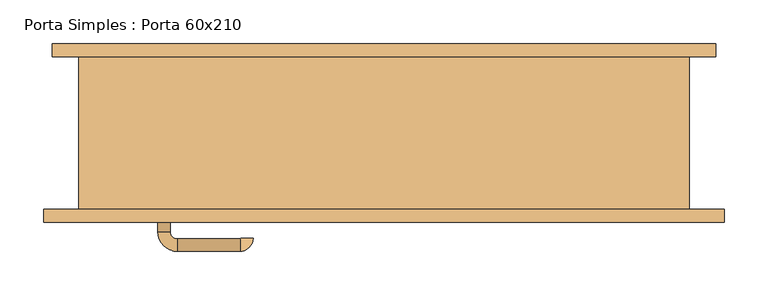
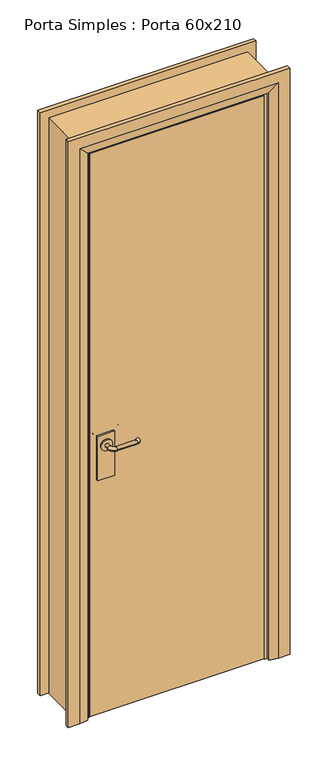
"""IFC4 building model written with IfcOpenShell, lengths in millimetres: door geometry, Porta Simples : Porta 60x210."""

from ifc_helpers import new_model, si_unit, point, frame, frame_2d, origin, place, context, project, spatial, polyline, circle_curve, ellipse_curve, trimmed, segment, composite_curve, outline, extrude, faceted_brep, source, transform, mapped, element, save
from ifc_brep_helpers import plane_surface, cylinder_surface, revolved_surface, advanced_brep


def porta_simples_porta_60x210_4542fb52(model_context):
    return source(origin(), model_context, "Body", "SolidModel", [
        extrude(outline(composite_curve([segment(trimmed(circle_curve(frame_2d((1050.0, -252.0)), 20.0), [point((1050.0, -272.0))], [point((1050.0, -232.0))], False, "CARTESIAN"), True, "CONTINUOUS"), segment(trimmed(circle_curve(frame_2d((1050.0, -252.0)), 20.0), [point((1050.0, -232.0))], [point((1050.0, -272.0))], False, "CARTESIAN"), True, "CONTINUOUS")], self_intersect=False)), frame((0.0, -46.3, 0.0), z_axis=(0.0, 1.0, 0.0), x_axis=(0.0, 0.0, 1.0)), (0.0, 0.0, 1.0), 4.5929895),
        advanced_brep(
        [(-245.0, -41.7070105, 1050.0), (-259.0, -41.7070105, 1050.0), (-245.0, -26.3, 1050.0), (-259.0, -26.3, 1050.0), (-237.0, -4.3, 1050.0), (-237.0, -18.3, 1050.0), (-165.0, -18.3, 1050.0), (-165.0, -4.3, 1050.0), (-164.0, -19.3, 1050.0), (-150.0, -19.3, 1050.0)],
        [
            (0, 1, circle_curve(frame((-252.0, -41.7070105, 1050.0), z_axis=(0.0, -1.0, 0.0), x_axis=(-1.0, 0.0, 0.0)), 7.0)),
            (1, 0, circle_curve(frame((-252.0, -41.7070105, 1050.0), z_axis=(0.0, -1.0, 0.0), x_axis=(-1.0, 0.0, 0.0)), 7.0)),
            (0, 2),
            (2, 3, circle_curve(frame((-252.0, -26.3, 1050.0), z_axis=(0.0, -1.0, 0.0), x_axis=(-1.0, 0.0, 0.0)), 7.0)),
            (3, 1),
            (3, 2, circle_curve(frame((-252.0, -26.3, 1050.0), z_axis=(0.0, -1.0, 0.0), x_axis=(-1.0, 0.0, 0.0)), 7.0)),
            (4, 3, circle_curve(frame((-237.0, -26.3, 1050.0), z_axis=(0.0, 0.0, 1.0), x_axis=(-1.0, 0.0, 0.0)), 22.0)),
            (2, 5, circle_curve(frame((-237.0, -26.3, 1050.0), z_axis=(0.0, 0.0, -1.0), x_axis=(-1.0, 0.0, 0.0)), 8.0)),
            (5, 4, circle_curve(frame((-237.0, -11.3, 1050.0), z_axis=(-1.0, 0.0, 0.0), x_axis=(0.0, 1.0, 0.0)), 7.0)),
            (4, 5, circle_curve(frame((-237.0, -11.3, 1050.0), z_axis=(-1.0, 0.0, 0.0), x_axis=(0.0, 1.0, 0.0)), 7.0)),
            (5, 6),
            (6, 7, circle_curve(frame((-165.0, -11.3, 1050.0), z_axis=(-1.0, 0.0, 0.0), x_axis=(0.0, 1.0, 0.0)), 7.0)),
            (7, 4),
            (7, 6, circle_curve(frame((-165.0, -11.3, 1050.0), z_axis=(-1.0, 0.0, 0.0), x_axis=(0.0, 1.0, 0.0)), 7.0)),
            (8, 9, circle_curve(frame((-157.0, -19.3, 1050.0), z_axis=(0.0, -1.0, 0.0), x_axis=(1.0, 0.0, 0.0)), 7.0)),
            (9, 8, circle_curve(frame((-157.0, -19.3, 1050.0), z_axis=(0.0, -1.0, 0.0), x_axis=(1.0, 0.0, 0.0)), 7.0)),
            (9, 7, circle_curve(frame((-165.0, -19.3, 1050.0), z_axis=(0.0, 0.0, 1.0), x_axis=(0.0, 1.0, 0.0)), 15.0)),
            (6, 8, circle_curve(frame((-165.0, -19.3, 1050.0), z_axis=(0.0, 0.0, -1.0), x_axis=(0.0, 1.0, 0.0)), 1.0)),
        ],
        [
            plane_surface(frame((-252.0, -41.7070105, 1050.0), z_axis=(0.0, -1.0, 0.0), x_axis=(0.0, 0.0, 1.0))),
            cylinder_surface(frame((-252.0, -41.7070105, 1050.0), z_axis=(0.0, -1.0, 0.0), x_axis=(-1.0, 0.0, 0.0)), 7.0),
            revolved_surface(trimmed(ellipse_curve(frame((-252.0, -26.3, 1050.0), z_axis=(0.0, -1.0, 0.0), x_axis=(-1.0, 0.0, 0.0)), 7.0, 7.0), [point((-245.0, -26.3, 1050.0))], [point((-259.0, -26.3, 1050.0))], True, "CARTESIAN"), (-237.0, -26.3, 1050.0), (0.0, 0.0, -1.0)),
            revolved_surface(trimmed(ellipse_curve(frame((-252.0, -26.3, 1050.0), z_axis=(0.0, -1.0, 0.0), x_axis=(-1.0, 0.0, 0.0)), 7.0, 7.0), [point((-259.0, -26.3, 1050.0))], [point((-245.0, -26.3, 1050.0))], True, "CARTESIAN"), (-237.0, -26.3, 1050.0), (0.0, 0.0, -1.0)),
            cylinder_surface(frame((-237.0, -11.3, 1050.0), z_axis=(-1.0, 0.0, 0.0), x_axis=(0.0, 1.0, 0.0)), 7.0),
            plane_surface(frame((-157.0, -19.3, 1050.0), z_axis=(0.0, -1.0, 0.0), x_axis=(0.0, 0.0, 1.0))),
            revolved_surface(trimmed(ellipse_curve(frame((-165.0, -11.3, 1050.0), z_axis=(-1.0, 0.0, 0.0), x_axis=(0.0, 1.0, 0.0)), 7.0, 7.0), [point((-165.0, -18.3, 1050.0))], [point((-165.0, -4.3, 1050.0))], True, "CARTESIAN"), (-165.0, -19.3, 1050.0), (0.0, 0.0, -1.0)),
            revolved_surface(trimmed(ellipse_curve(frame((-165.0, -11.3, 1050.0), z_axis=(-1.0, 0.0, 0.0), x_axis=(0.0, 1.0, 0.0)), 7.0, 7.0), [point((-165.0, -4.3, 1050.0))], [point((-165.0, -18.3, 1050.0))], True, "CARTESIAN"), (-165.0, -19.3, 1050.0), (0.0, 0.0, -1.0)),
        ],
        [
            (0, [[1, 2]]),
            (1, [[-1, 3, 4, 5]]),
            (1, [[-2, -5, 6, -3]]),
            (2, [[7, -4, 8, 9]]),
            (3, [[-8, -6, -7, 10]]),
            (4, [[-9, 11, 12, 13]]),
            (4, [[-10, -13, 14, -11]]),
            (5, [[15, 16]]),
            (6, [[17, -12, 18, -16]]),
            (7, [[-18, -14, -17, -15]]),
        ],
    ),
        extrude(outline(polyline([(-222.0, -52.3), (-282.0, -52.3), (-282.0, -46.3), (-222.0, -46.3), (-222.0, -52.3)])), frame((0.0, 0.0, 925.0), z_axis=(0.0, 0.0, 1.0), x_axis=(1.0, 0.0, 0.0)), (0.0, 0.0, 1.0), 165.0),
        extrude(outline(composite_curve([segment(trimmed(circle_curve(frame_2d((1050.0, -252.0)), 20.0), [point((1050.0, -272.0))], [point((1050.0, -232.0))], False, "CARTESIAN"), True, "CONTINUOUS"), segment(trimmed(circle_curve(frame_2d((1050.0, -252.0)), 20.0), [point((1050.0, -232.0))], [point((1050.0, -272.0))], False, "CARTESIAN"), True, "CONTINUOUS")], self_intersect=False)), frame((0.0, -97.8929895, 0.0), z_axis=(0.0, 1.0, 0.0), x_axis=(0.0, 0.0, 1.0)), (0.0, 0.0, 1.0), 4.5929895),
        advanced_brep(
        [(-245.0, -97.8929895, 1050.0), (-259.0, -97.8929895, 1050.0), (-259.0, -113.3, 1050.0), (-245.0, -113.3, 1050.0), (-237.0, -135.3, 1050.0), (-237.0, -121.3, 1050.0), (-165.0, -135.3, 1050.0), (-165.0, -121.3, 1050.0), (-164.0, -120.3, 1050.0), (-150.0, -120.3, 1050.0)],
        [
            (0, 1, circle_curve(frame((-252.0, -97.8929895, 1050.0), z_axis=(0.0, 1.0, 0.0), x_axis=(-1.0, 0.0, 0.0)), 7.0)),
            (1, 0, circle_curve(frame((-252.0, -97.8929895, 1050.0), z_axis=(0.0, 1.0, 0.0), x_axis=(-1.0, 0.0, 0.0)), 7.0)),
            (1, 2),
            (2, 3, circle_curve(frame((-252.0, -113.3, 1050.0), z_axis=(0.0, 1.0, 0.0), x_axis=(-1.0, 0.0, 0.0)), 7.0)),
            (3, 0),
            (3, 2, circle_curve(frame((-252.0, -113.3, 1050.0), z_axis=(0.0, 1.0, 0.0), x_axis=(-1.0, 0.0, 0.0)), 7.0)),
            (4, 5, circle_curve(frame((-237.0, -128.3, 1050.0), z_axis=(-1.0, 0.0, 0.0), x_axis=(0.0, -1.0, 0.0)), 7.0)),
            (5, 3, circle_curve(frame((-237.0, -113.3, 1050.0), z_axis=(0.0, 0.0, -1.0), x_axis=(-1.0, 0.0, 0.0)), 8.0)),
            (2, 4, circle_curve(frame((-237.0, -113.3, 1050.0), z_axis=(0.0, 0.0, 1.0), x_axis=(-1.0, 0.0, 0.0)), 22.0)),
            (5, 4, circle_curve(frame((-237.0, -128.3, 1050.0), z_axis=(-1.0, 0.0, 0.0), x_axis=(0.0, -1.0, 0.0)), 7.0)),
            (4, 6),
            (6, 7, circle_curve(frame((-165.0, -128.3, 1050.0), z_axis=(-1.0, 0.0, 0.0), x_axis=(0.0, -1.0, 0.0)), 7.0)),
            (7, 5),
            (7, 6, circle_curve(frame((-165.0, -128.3, 1050.0), z_axis=(-1.0, 0.0, 0.0), x_axis=(0.0, -1.0, 0.0)), 7.0)),
            (8, 9, circle_curve(frame((-157.0, -120.3, 1050.0), z_axis=(0.0, 1.0, 0.0), x_axis=(1.0, 0.0, 0.0)), 7.0)),
            (9, 8, circle_curve(frame((-157.0, -120.3, 1050.0), z_axis=(0.0, 1.0, 0.0), x_axis=(1.0, 0.0, 0.0)), 7.0)),
            (8, 7, circle_curve(frame((-165.0, -120.3, 1050.0), z_axis=(0.0, 0.0, -1.0), x_axis=(0.0, -1.0, 0.0)), 1.0)),
            (6, 9, circle_curve(frame((-165.0, -120.3, 1050.0), z_axis=(0.0, 0.0, 1.0), x_axis=(0.0, -1.0, 0.0)), 15.0)),
        ],
        [
            plane_surface(frame((-252.0, -97.8929895, 1050.0), z_axis=(0.0, 1.0, 0.0), x_axis=(0.0, 0.0, 1.0))),
            cylinder_surface(frame((-252.0, -97.8929895, 1050.0), z_axis=(0.0, 1.0, 0.0), x_axis=(-1.0, 0.0, 0.0)), 7.0),
            revolved_surface(trimmed(ellipse_curve(frame((-252.0, -113.3, 1050.0), z_axis=(0.0, -1.0, 0.0), x_axis=(-1.0, 0.0, 0.0)), 7.0, 7.0), [point((-245.0, -113.3, 1050.0))], [point((-259.0, -113.3, 1050.0))], True, "CARTESIAN"), (-237.0, -113.3, 1050.0), (0.0, 0.0, -1.0)),
            revolved_surface(trimmed(ellipse_curve(frame((-252.0, -113.3, 1050.0), z_axis=(0.0, -1.0, 0.0), x_axis=(-1.0, 0.0, 0.0)), 7.0, 7.0), [point((-259.0, -113.3, 1050.0))], [point((-245.0, -113.3, 1050.0))], True, "CARTESIAN"), (-237.0, -113.3, 1050.0), (0.0, 0.0, -1.0)),
            cylinder_surface(frame((-237.0, -128.3, 1050.0), z_axis=(-1.0, 0.0, 0.0), x_axis=(0.0, -1.0, 0.0)), 7.0),
            plane_surface(frame((-157.0, -120.3, 1050.0), z_axis=(0.0, 1.0, 0.0), x_axis=(0.0, 0.0, 1.0))),
            revolved_surface(trimmed(ellipse_curve(frame((-165.0, -128.3, 1050.0), z_axis=(1.0, 0.0, 0.0), x_axis=(0.0, -1.0, 0.0)), 7.0, 7.0), [point((-165.0, -121.3, 1050.0))], [point((-165.0, -135.3, 1050.0))], True, "CARTESIAN"), (-165.0, -120.3, 1050.0), (0.0, 0.0, -1.0)),
            revolved_surface(trimmed(ellipse_curve(frame((-165.0, -128.3, 1050.0), z_axis=(1.0, 0.0, 0.0), x_axis=(0.0, -1.0, 0.0)), 7.0, 7.0), [point((-165.0, -135.3, 1050.0))], [point((-165.0, -121.3, 1050.0))], True, "CARTESIAN"), (-165.0, -120.3, 1050.0), (0.0, 0.0, -1.0)),
        ],
        [
            (0, [[1, 2]]),
            (1, [[3, 4, 5, -2]]),
            (1, [[-5, 6, -3, -1]]),
            (2, [[7, 8, -4, 9]]),
            (3, [[10, -9, -6, -8]]),
            (4, [[11, 12, 13, -7]]),
            (4, [[-13, 14, -11, -10]]),
            (5, [[15, 16]]),
            (6, [[-15, 17, -12, 18]]),
            (7, [[-16, -18, -14, -17]]),
        ],
    ),
        extrude(outline(polyline([(-222.0, -87.3), (-222.0, -93.3), (-282.0, -93.3), (-282.0, -87.3), (-222.0, -87.3)])), frame((0.0, 0.0, 925.0), z_axis=(0.0, 0.0, 1.0), x_axis=(1.0, 0.0, 0.0)), (0.0, 0.0, 1.0), 165.0),
        extrude(outline(polyline([(307.0, -52.3), (307.0, -87.3), (-307.0, -87.3), (-307.0, -52.3), (307.0, -52.3)])), frame((0.0, 0.0, 53.0), z_axis=(0.0, 0.0, 1.0), x_axis=(1.0, 0.0, 0.0)), (0.0, 0.0, 1.0), 2094.0),
        faceted_brep([(380.0, 87.3, 50.0), (310.0, 87.3, 50.0), (310.0, 97.3, 50.0), (340.0, 102.3, 50.0), (380.0, 102.3, 50.0), (380.0, 102.3, 2220.0), (380.0, 87.3, 2220.0), (340.0, 102.3, 2180.0), (-340.0, 102.3, 2180.0), (-340.0, 102.3, 50.0), (-380.0, 102.3, 50.0), (-380.0, 102.3, 2220.0), (310.0, 97.3, 2150.0), (310.0, 87.3, 2150.0), (-380.0, 87.3, 2220.0), (-380.0, 87.3, 50.0), (-310.0, 87.3, 50.0), (-310.0, 87.3, 2150.0), (-310.0, 97.3, 50.0), (-310.0, 97.3, 2150.0)], [[[0, 1, 2, 3, 4]], [[4, 5, 6, 0]], [[3, 7, 8, 9, 10, 11, 5, 4]], [[2, 12, 7, 3]], [[1, 13, 12, 2]], [[0, 6, 14, 15, 16, 17, 13, 1]], [[17, 16, 18, 19]], [[15, 10, 9, 18, 16]], [[11, 10, 15, 14]], [[19, 18, 9, 8]], [[13, 17, 19, 12]], [[5, 11, 14, 6]], [[12, 19, 8, 7]]]),
        faceted_brep([(390.0, -87.3, 50.0), (390.0, -102.3, 50.0), (350.0, -102.3, 50.0), (320.0, -97.3, 50.0), (320.0, -87.3, 50.0), (320.0, -87.3, 2160.0), (-320.0, -87.3, 2160.0), (-320.0, -87.3, 50.0), (-390.0, -87.3, 50.0), (-390.0, -87.3, 2230.0), (390.0, -87.3, 2230.0), (320.0, -97.3, 2160.0), (350.0, -102.3, 2190.0), (390.0, -102.3, 2230.0), (-390.0, -102.3, 2230.0), (-390.0, -102.3, 50.0), (-350.0, -102.3, 50.0), (-350.0, -102.3, 2190.0), (-320.0, -97.3, 50.0), (-320.0, -97.3, 2160.0)], [[[0, 1, 2, 3, 4]], [[4, 5, 6, 7, 8, 9, 10, 0]], [[3, 11, 5, 4]], [[2, 12, 11, 3]], [[1, 13, 14, 15, 16, 17, 12, 2]], [[0, 10, 13, 1]], [[9, 8, 15, 14]], [[8, 7, 18, 16, 15]], [[19, 18, 7, 6]], [[17, 16, 18, 19]], [[11, 19, 6, 5]], [[10, 9, 14, 13]], [[12, 17, 19, 11]]]),
        faceted_brep([(-310.0, -87.3, 50.0), (-350.0, -87.3, 50.0), (-350.0, 87.3, 50.0), (-300.0, 87.3, 50.0), (-300.0, -49.3, 50.0), (-310.0, -49.3, 50.0), (-310.0, -49.3, 2150.0), (-310.0, -87.3, 2150.0), (-300.0, -49.3, 2140.0), (-300.0, 87.3, 2140.0), (-350.0, 87.3, 2190.0), (-350.0, -87.3, 2190.0), (310.0, -87.3, 50.0), (310.0, -49.3, 50.0), (300.0, -49.3, 50.0), (300.0, 87.3, 50.0), (350.0, 87.3, 50.0), (350.0, -87.3, 50.0), (310.0, -87.3, 2150.0), (350.0, -87.3, 2190.0), (350.0, 87.3, 2190.0), (300.0, 87.3, 2140.0), (300.0, -49.3, 2140.0), (310.0, -49.3, 2150.0)], [[[0, 1, 2, 3, 4, 5]], [[5, 6, 7, 0]], [[4, 8, 6, 5]], [[3, 9, 8, 4]], [[2, 10, 9, 3]], [[1, 11, 10, 2]], [[0, 7, 11, 1]], [[12, 13, 14, 15, 16, 17]], [[18, 12, 17, 19]], [[19, 17, 16, 20]], [[20, 16, 15, 21]], [[21, 15, 14, 22]], [[22, 14, 13, 23]], [[23, 13, 12, 18]], [[6, 23, 18, 7]], [[8, 22, 23, 6]], [[9, 21, 22, 8]], [[10, 20, 21, 9]], [[11, 19, 20, 10]], [[7, 18, 19, 11]]]),
    ])


if __name__ == "__main__":
    model = new_model("IFC4")
    model_context = context("Model", 3, world=origin())
    ifc_project = project(units=[si_unit("LENGTHUNIT", "METRE", prefix="MILLI")], contexts=[model_context])
    site = spatial("IfcSite", under=ifc_project)
    building = spatial("IfcBuilding", under=site)
    placement = place(None, origin())
    porta_simples_porta_60x210_shape = porta_simples_porta_60x210_4542fb52(model_context)
    element("IfcDoor", 1, ObjectType="Porta Simples : Porta 60x210", at=placement, inside=building, context=model_context, shape_type="MappedRepresentation", body=[
        mapped(porta_simples_porta_60x210_shape, transform((0.0, 0.0, 0.0), x_axis=(1.0, 0.0, 0.0), y_axis=(0.0, 1.0, 0.0), z_axis=(0.0, 0.0, 1.0))),
    ])
    save(model, "model.ifc")

# Revit data of these elements
# Type "Porta Simples : Porta 60x210"
#   Type Mark = "51"
#   SINAPI = ""
#   Analytic Construction = "<Nenhum>"
#   Maçaneta [instance default] = ""
#   Fechadura [instance default] = ""
#   Vão Luz (somente para informação) = 0.58 m
#   Tolerância Folha Vertical = 0.003 m
#   Módulo Básico M = 0.10 m
#   Largura de Coordenação Modular Largura CM = 0.70 m
#   Rough Width = 0.70 m
#   Deslocamento da Horizontal da Folha = 0.00 m
#   Altura de Coordenação Modular Largura CM = 2.20 m
#   Rough Height = 2.20 m
#   Altura Nominal = 2.09 m
#   Ajuste de Coordenação Topo AC Topo = 0.01 m
#   Ajuste de Coordenação Base AC Base = 0.05 m
#   Ajuste de Coordenação AC = 0.01 m
#   Tolerância Folha Horizontal = 0.003 m
#   Largura Folha (somente para informação) = 0.594 m
#   Espessura Folha = 0.035 m
#   Maçaneta - Distância da Folha = 0.055 m
#   Maçaneta - Altura = 1.00 m
#   Largura Nominal (Largura Mn) = 0.62 m
#   Distância do Nível = 0.003 m
#   Aduela Interna Espessura = 0.04 m
#   Aduela Externa Espessura = 0.05 m
#   Altura Folha (somente para informação) = 2.074 m
#   Height = 2.14 m
#   Width = 0.68 m
#   Número de Módulos Básicos nM Largura = 7
#   Número de Módulos Básicos nM Altura = 22
#   Marco Metálico = no
#   Aduela de Madeira = no
#   Aduela Metálica de Canto = no
#   Guarnição Reta = no
#   Guarnição Chanfrada = yes
#   Batente - Material [instance default] = none
#   Painel - Material [instance default] = none
#   Construction Type = (empty or 0)
#   Model = ""
#   Function = (empty or 0)
#   Description = (empty or 0)
#   Wall Closure = (empty or 0)
#   Assembly Code = ""
# Element 1 (IfcDoor, "Porta Simples : Porta 60x210")
#   Materials on its faces: "Porta - Maçaneta"
# Materials
#   "Porta - Maçaneta": class "Diversos", colour RGB 0 0 0, transparency 0
